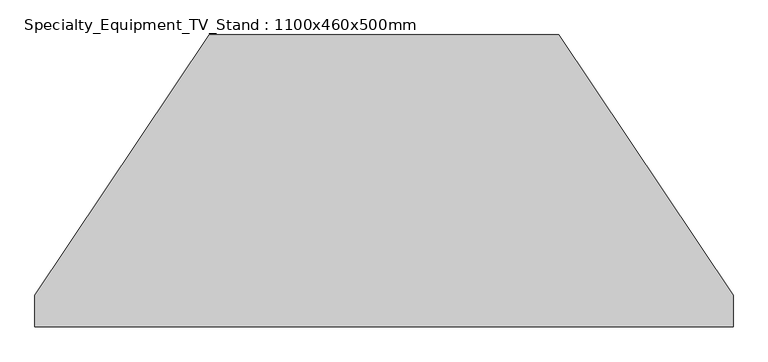
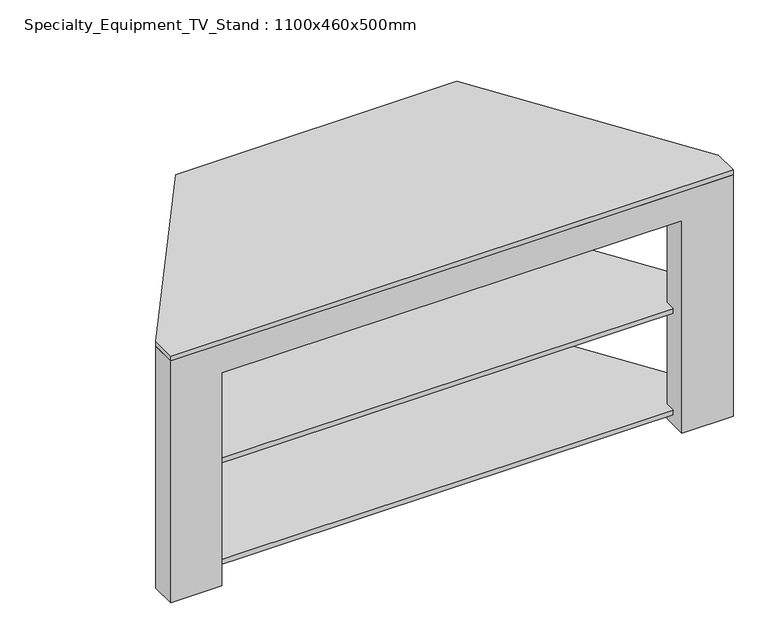
"""IFC4 building model written with IfcOpenShell, lengths in millimetres: proxy geometry, Specialty_Equipment_TV_Stand : 1100x460x500mm."""

import ifcopenshell
import ifcopenshell.guid

model = None  # the IFC model being written
_history = None  # IfcOwnerHistory: only IFC2X3 demands one
_inside = {}  # id of a spatial element -> (the spatial element, [elements in it])
_under = {}  # id of a project, library or spatial element -> (it, [spatial elements below it])
_declared = {}  # id of a project -> (the project, [libraries it declares])
_typed = {}  # id of a type object -> (the type object, [elements of that type])
_made_of = {}  # id of a material, layer set ... -> (it, [elements and type objects made of it])


def new_model(schema):
    """Start an empty IFC model of exactly this schema.

    Asked for "IFC4X3", IfcOpenShell would pick the latest addendum, in which some entities
    have other attributes; the version numbers below select the first issue.
    IFC2X3 requires an IfcOwnerHistory on every rooted entity: one is made here for all.
    """
    global model, _history
    if schema == "IFC4X3":
        model = ifcopenshell.file(schema_version=(4, 3, 0, 0))
    else:
        model = ifcopenshell.file(schema=schema)
    _inside.clear()
    _under.clear()
    _declared.clear()
    _typed.clear()
    _made_of.clear()
    _history = None
    if model.schema == "IFC2X3":
        org = make("IfcOrganization", Name="unknown")
        user = make(
            "IfcPersonAndOrganization",
            ThePerson=make("IfcPerson", FamilyName="unknown"),
            TheOrganization=org,
        )
        app = make(
            "IfcApplication",
            ApplicationDeveloper=org,
            Version="unknown",
            ApplicationFullName="unknown",
            ApplicationIdentifier="unknown",
        )
        _history = make(
            "IfcOwnerHistory",
            OwningUser=user,
            OwningApplication=app,
            ChangeAction="ADDED",
            CreationDate=0,
        )
    return model


def make(cls, **values):
    """One entity of the class cls with the attributes given. An attribute that is None is left unset."""
    return model.create_entity(
        cls, **{name: value for name, value in values.items() if value is not None}
    )


def rooted(cls, **values):
    """An entity with a GlobalId (a new one), such as an element, a storey or a relation."""
    return make(cls, GlobalId=ifcopenshell.guid.new(), OwnerHistory=_history, **values)


def si_unit(unit_type, name, prefix=None):
    """IfcSIUnit, for example si_unit("LENGTHUNIT", "METRE", prefix="MILLI")."""
    return make("IfcSIUnit", UnitType=unit_type, Prefix=prefix, Name=name)


def assignment(units):
    """IfcUnitAssignment: the units of a project."""
    return None if units is None else make("IfcUnitAssignment", Units=units)


def point(xyz):
    """IfcCartesianPoint."""
    return None if xyz is None else make("IfcCartesianPoint", Coordinates=xyz)


def direction(xyz):
    """IfcDirection."""
    return None if xyz is None else make("IfcDirection", DirectionRatios=xyz)


def frame(location, z_axis=None, x_axis=None):
    """IfcAxis2Placement3D, a coordinate frame: its origin and axes. An axis left out is left unset."""
    return make(
        "IfcAxis2Placement3D",
        Location=point(location),
        Axis=direction(z_axis),
        RefDirection=direction(x_axis),
    )


def frame_2d(location, x_axis=None):
    """IfcAxis2Placement2D, a coordinate frame in the plane: its origin and x axis."""
    return make(
        "IfcAxis2Placement2D", Location=point(location), RefDirection=direction(x_axis)
    )


def origin():
    """The frame at (0, 0, 0) with its axes left unset."""
    return frame((0.0, 0.0, 0.0))


def place(relative_to, where):
    """IfcLocalPlacement: puts the frame where relative to a parent placement (None: the world)."""
    return make(
        "IfcLocalPlacement", PlacementRelTo=relative_to, RelativePlacement=where
    )


def context(
    kind, dimensions, precision=None, world=None, true_north=None, identifier=None
):
    """IfcGeometricRepresentationContext, for example the 3D "Model" context."""
    return make(
        "IfcGeometricRepresentationContext",
        ContextIdentifier=identifier,
        ContextType=kind,
        CoordinateSpaceDimension=dimensions,
        Precision=precision,
        WorldCoordinateSystem=world,
        TrueNorth=true_north,
    )


def project(units=None, contexts=None):
    """IfcProject with its units and contexts."""
    return rooted(
        "IfcProject",
        Name="project",
        RepresentationContexts=contexts,
        UnitsInContext=assignment(units),
    )


def spatial(cls, under=None, at=None, **own):
    """A site, building, storey or space (cls), placed at a placement, below another one or the project."""
    s = rooted(cls, ObjectPlacement=at, **own)
    if under is not None:
        _under.setdefault(under.id(), (under, []))[1].append(s)
    return s


def polyline(points):
    """IfcPolyline through the points."""
    return make("IfcPolyline", Points=[point(p) for p in points])


def circle_curve(where, radius):
    """IfcCircle in the frame where."""
    return make("IfcCircle", Position=where, Radius=radius)


def trimmed(basis, trim1, trim2, sense, master):
    """IfcTrimmedCurve: the piece of a basis curve between two trims."""
    return make(
        "IfcTrimmedCurve",
        BasisCurve=basis,
        Trim1=trim1,
        Trim2=trim2,
        SenseAgreement=sense,
        MasterRepresentation=master,
    )


def segment(curve, same_sense, transition):
    """IfcCompositeCurveSegment."""
    return make(
        "IfcCompositeCurveSegment",
        Transition=transition,
        SameSense=same_sense,
        ParentCurve=curve,
    )


def composite_curve(segments, self_intersect=None):
    """IfcCompositeCurve: segments joined end to end."""
    return make("IfcCompositeCurve", Segments=segments, SelfIntersect=self_intersect)


def outline(outer, holes=None, kind="AREA"):
    """IfcArbitraryClosedProfileDef: a profile drawn as a closed curve; with holes, ...WithVoids."""
    if holes is None:
        return make("IfcArbitraryClosedProfileDef", ProfileType=kind, OuterCurve=outer)
    return make(
        "IfcArbitraryProfileDefWithVoids",
        ProfileType=kind,
        OuterCurve=outer,
        InnerCurves=holes,
    )


def extrude(swept, where, along, depth):
    """IfcExtrudedAreaSolid: the profile swept, set in the frame where, extruded along a direction by depth."""
    return make(
        "IfcExtrudedAreaSolid",
        SweptArea=swept,
        Position=where,
        ExtrudedDirection=direction(along),
        Depth=depth,
    )


def faces_of(points, faces, orient=None, outer=None):
    """IfcFace entities. A face is a list of loops; a loop is a list of indices into points, from 0.

    orient and outer hold one flag for each loop. By default every Orientation is true, the
    first loop of a face is its IfcFaceOuterBound and the others are IfcFaceBound.
    """
    made = []
    for i, loops in enumerate(faces):
        bounds = []
        for j, loop in enumerate(loops):
            is_outer = j == 0 if outer is None else outer[i][j]
            bounds.append(
                make(
                    "IfcFaceOuterBound" if is_outer else "IfcFaceBound",
                    Bound=make("IfcPolyLoop", Polygon=[points[k] for k in loop]),
                    Orientation=True if orient is None else orient[i][j],
                )
            )
        made.append(make("IfcFace", Bounds=bounds))
    return made


def faceted_brep(points, faces, orient=None, outer=None, voids=None):
    """IfcFacetedBrep: a solid bounded by flat faces; with voids (closed shells), ...WithVoids."""
    shared = [point(p) for p in points]
    hull = make("IfcClosedShell", CfsFaces=faces_of(shared, faces, orient, outer))
    if voids is None:
        return make("IfcFacetedBrep", Outer=hull)
    return make(
        "IfcFacetedBrepWithVoids",
        Outer=hull,
        Voids=[
            make(cls, CfsFaces=faces_of(shared, fs, o, b)) for cls, fs, o, b in voids
        ],
    )


def shape(context_of_items, identifier, shape_type, items):
    """IfcShapeRepresentation: the items that make up one representation, for example the "Body"."""
    return make(
        "IfcShapeRepresentation",
        ContextOfItems=context_of_items,
        RepresentationIdentifier=identifier,
        RepresentationType=shape_type,
        Items=items,
    )


def source(mapping_origin, context_of_items, identifier, shape_type, items):
    """IfcRepresentationMap: a shape defined once, which mapped items show again and again."""
    return make(
        "IfcRepresentationMap",
        MappingOrigin=mapping_origin,
        MappedRepresentation=shape(context_of_items, identifier, shape_type, items),
    )


def transform(
    local_origin,
    x_axis=None,
    y_axis=None,
    z_axis=None,
    scale=None,
    scale2=None,
    scale3=None,
    uniform=True,
):
    """IfcCartesianTransformationOperator3D, or its non-uniform kind. x_axis, y_axis, z_axis: its Axis1, 2, 3."""
    if uniform:
        return make(
            "IfcCartesianTransformationOperator3D",
            Axis1=direction(x_axis),
            Axis2=direction(y_axis),
            LocalOrigin=point(local_origin),
            Scale=scale,
            Axis3=direction(z_axis),
        )
    return make(
        "IfcCartesianTransformationOperator3DnonUniform",
        Axis1=direction(x_axis),
        Axis2=direction(y_axis),
        LocalOrigin=point(local_origin),
        Scale=scale,
        Axis3=direction(z_axis),
        Scale2=scale2,
        Scale3=scale3,
    )


def mapped(mapping_source, mapping_target):
    """IfcMappedItem: shows the shape of a source again, moved by a transform."""
    return make(
        "IfcMappedItem", MappingSource=mapping_source, MappingTarget=mapping_target
    )


def made_of(thing, what):
    """Note that an element or type object is made of a material, layer set ...; save() writes the relation."""
    if what is not None:
        _made_of.setdefault(what.id(), (what, []))[1].append(thing)
    return thing


def element(
    cls,
    number,
    at=None,
    inside=None,
    cuts=None,
    type_object=None,
    material=None,
    context=None,
    identifier="Body",
    shape_type=None,
    held_by="IfcProductDefinitionShape",
    body=None,
    shapes=None,
    **own,
):
    """One element of the class cls, such as IfcWall. Its Tag is "e" and its number.

    at: its placement. inside: the storey or other place that contains it. cuts: it is an
    opening in that element (IfcRelVoidsElement). A single representation is given by context,
    identifier, shape_type and body (its items); several are given by shapes. held_by: the class
    of the entity that holds the representations. save() writes the other relations.
    """
    e = rooted(cls, Tag="e%d" % number, ObjectPlacement=at, **own)
    if body is not None:
        shapes = [shape(context, identifier, shape_type, body)]
    if shapes is not None:
        e.Representation = make(held_by, Representations=shapes)
    if inside is not None:
        _inside.setdefault(inside.id(), (inside, []))[1].append(e)
    if cuts is not None:
        rooted(
            "IfcRelVoidsElement", RelatingBuildingElement=cuts, RelatedOpeningElement=e
        )
    if type_object is not None:
        _typed.setdefault(type_object.id(), (type_object, []))[1].append(e)
    return made_of(e, material)


def aggregate(whole, parts):
    """IfcRelAggregates: a whole, such as a stair, and the parts it consists of."""
    return rooted("IfcRelAggregates", RelatingObject=whole, RelatedObjects=parts)


def save(model, path):
    """Write the relations noted so far, then the file.

    IfcRelAggregates (storeys below a building ...), IfcRelContainedInSpatialStructure (elements
    in a storey), IfcRelDefinesByType, IfcRelAssociatesMaterial and IfcRelDeclares: one each for
    every whole, place, type object, material and project.
    """
    for whole, parts in _under.values():
        aggregate(whole, parts)
    for where, things in _inside.values():
        rooted(
            "IfcRelContainedInSpatialStructure",
            RelatedElements=things,
            RelatingStructure=where,
        )
    for kind, things in _typed.values():
        rooted("IfcRelDefinesByType", RelatedObjects=things, RelatingType=kind)
    for what, things in _made_of.values():
        rooted("IfcRelAssociatesMaterial", RelatedObjects=things, RelatingMaterial=what)
    for by, libraries in _declared.values():
        rooted("IfcRelDeclares", RelatingContext=by, RelatedDefinitions=libraries)
    model.write(path)


def specialty_equipment_tv_stand_1100x460x500mm_40ec15d9(model_context):
    return source(origin(), model_context, "Body", "SolidModel", [
        extrude(outline(polyline([(420.3099533, -30.0), (625.1880021, -335.4545455), (625.1880021, -430.0), (-374.8119979, -430.0), (-374.8119979, -335.4545455), (-169.9339492, -30.0), (420.3099533, -30.0)])), frame((0.0, 0.0, 20.0), z_axis=(0.0, 0.0, 1.0), x_axis=(1.0, 0.0, 0.0)), (0.0, 0.0, 1.0), 10.0),
        extrude(outline(polyline([(420.3099533, -30.0), (625.1880021, -335.4545455), (625.1880021, -430.0), (-374.8119979, -430.0), (-374.8119979, -335.4545455), (-169.9339492, -30.0), (420.3099533, -30.0)])), frame((0.0, 0.0, 230.0), z_axis=(0.0, 0.0, 1.0), x_axis=(1.0, 0.0, 0.0)), (0.0, 0.0, 1.0), 10.0),
        extrude(outline(polyline([(400.1880021, 0.0), (675.1880021, -410.0), (675.1880021, -460.0), (-424.8119979, -460.0), (-424.8119979, -410.0), (-149.8119979, 0.0), (400.1880021, 0.0)])), frame((0.0, 0.0, 500.0), z_axis=(0.0, 0.0, 1.0), x_axis=(1.0, 0.0, 0.0)), (0.0, 0.0, 1.0), 10.0),
        extrude(outline(polyline([(-50.0, 500.0), (0.0, 500.0), (0.0, 0.0), (-50.0, 0.0), (-50.0, 20.0), (-30.0, 20.0), (-30.0, 30.0), (-50.0, 30.0), (-50.0, 230.0), (-30.0, 230.0), (-30.0, 240.0), (-50.0, 240.0), (-50.0, 500.0)])), frame((-149.8119979, 0.0, 0.0), z_axis=(1.0, 0.0, 0.0), x_axis=(0.0, 1.0, 0.0)), (0.0, 0.0, 1.0), 100.0),
        extrude(outline(polyline([(-50.0, 500.0), (0.0, 500.0), (0.0, 0.0), (-50.0, 0.0), (-50.0, 20.0), (-30.0, 20.0), (-30.0, 30.0), (-50.0, 30.0), (-50.0, 230.0), (-30.0, 230.0), (-30.0, 240.0), (-50.0, 240.0), (-50.0, 500.0)])), frame((300.1880021, 0.0, 0.0), z_axis=(1.0, 0.0, 0.0), x_axis=(0.0, 1.0, 0.0)), (0.0, 0.0, 1.0), 100.0),
        faceted_brep([(-424.8119979, -460.0, 0.0), (-324.8119979, -460.0, 0.0), (-324.8119979, -460.0, 440.0), (575.1880021, -460.0, 440.0), (575.1880021, -460.0, 0.0), (675.1880021, -460.0, 0.0), (675.1880021, -460.0, 500.0), (-424.8119979, -460.0, 500.0), (-424.8119979, -410.0, 0.0), (-424.8119979, -410.0, 500.0), (675.1880021, -410.0, 500.0), (675.1880021, -410.0, 0.0), (575.1880021, -410.0, 0.0), (575.1880021, -410.0, 20.0), (625.1880021, -410.0, 20.0), (625.1880021, -410.0, 30.0), (575.1880021, -410.0, 30.0), (575.1880021, -410.0, 230.0), (625.1880021, -410.0, 230.0), (625.1880021, -410.0, 240.0), (575.1880021, -410.0, 240.0), (575.1880021, -410.0, 440.0), (-324.8119979, -410.0, 440.0), (-324.8119979, -410.0, 240.0), (-374.8119979, -410.0, 240.0), (-374.8119979, -410.0, 230.0), (-324.8119979, -410.0, 230.0), (-324.8119979, -410.0, 30.0), (-374.8119979, -410.0, 30.0), (-374.8119979, -410.0, 20.0), (-324.8119979, -410.0, 20.0), (-324.8119979, -410.0, 0.0), (-324.8119979, -430.0, 20.0), (-324.8119979, -430.0, 30.0), (-324.8119979, -430.0, 230.0), (-324.8119979, -430.0, 240.0), (575.1880021, -430.0, 240.0), (575.1880021, -430.0, 230.0), (575.1880021, -430.0, 30.0), (575.1880021, -430.0, 20.0), (625.1880021, -430.0, 240.0), (-374.8119979, -430.0, 240.0), (-374.8119979, -430.0, 230.0), (625.1880021, -430.0, 230.0), (625.1880021, -430.0, 30.0), (-374.8119979, -430.0, 30.0), (-374.8119979, -430.0, 20.0), (625.1880021, -430.0, 20.0)], [[[0, 1, 2, 3, 4, 5, 6, 7]], [[8, 9, 10, 11, 12, 13, 14, 15, 16, 17, 18, 19, 20, 21, 22, 23, 24, 25, 26, 27, 28, 29, 30, 31]], [[1, 0, 8, 31]], [[2, 1, 31, 30, 32, 33, 27, 26, 34, 35, 23, 22]], [[3, 2, 22, 21]], [[4, 3, 21, 20, 36, 37, 17, 16, 38, 39, 13, 12]], [[5, 4, 12, 11]], [[6, 5, 11, 10]], [[7, 6, 10, 9]], [[0, 7, 9, 8]], [[19, 40, 36, 20]], [[35, 41, 24, 23]], [[25, 42, 34, 26]], [[37, 43, 18, 17]], [[41, 42, 25, 24]], [[42, 41, 35, 34]], [[40, 43, 37, 36]], [[43, 40, 19, 18]], [[15, 44, 38, 16]], [[33, 45, 28, 27]], [[29, 46, 32, 30]], [[39, 47, 14, 13]], [[45, 46, 29, 28]], [[46, 45, 33, 32]], [[44, 47, 39, 38]], [[47, 44, 15, 14]]]),
        extrude(outline(polyline([(0.0, 300.1880021), (500.0, 300.1880021), (500.0, -49.8119979), (0.0, -49.8119979), (0.0, 300.1880021)]), holes=[composite_curve([segment(polyline([(245.0, 145.1700818), (245.0, 105.2059224)]), True, "CONTINUOUS"), segment(trimmed(circle_curve(frame_2d((257.5, 105.2059224)), 12.5), [point((245.0, 105.2059224))], [point((270.0, 105.2059224))], True, "CARTESIAN"), True, "CONTINUOUS"), segment(polyline([(270.0, 105.2059224), (270.0, 145.1700818)]), True, "CONTINUOUS"), segment(trimmed(circle_curve(frame_2d((257.5, 145.1700818)), 12.5), [point((270.0, 145.1700818))], [point((245.0, 145.1700818))], True, "CARTESIAN"), True, "CONTINUOUS")], self_intersect=False), composite_curve([segment(polyline([(35.0, 145.1880021), (35.0, 105.2059224)]), True, "CONTINUOUS"), segment(trimmed(circle_curve(frame_2d((47.5, 105.2059224)), 12.5), [point((35.0, 105.2059224))], [point((60.0, 105.2059224))], True, "CARTESIAN"), True, "CONTINUOUS"), segment(polyline([(60.0, 105.2059224), (60.0, 145.1880021)]), True, "CONTINUOUS"), segment(trimmed(circle_curve(frame_2d((47.5, 145.1880021)), 12.5), [point((60.0, 145.1880021))], [point((35.0, 145.1880021))], True, "CARTESIAN"), True, "CONTINUOUS")], self_intersect=False)]), frame((0.0, -30.0, 0.0), z_axis=(0.0, 1.0, 0.0), x_axis=(0.0, 0.0, 1.0)), (0.0, 0.0, 1.0), 10.0),
    ])


if __name__ == "__main__":
    model = new_model("IFC4")
    model_context = context("Model", 3, world=origin())
    ifc_project = project(units=[si_unit("LENGTHUNIT", "METRE", prefix="MILLI")], contexts=[model_context])
    site = spatial("IfcSite", under=ifc_project)
    building = spatial("IfcBuilding", under=site)
    placement = place(None, origin())
    specialty_equipment_tv_stand_1100x460x500mm_shape = specialty_equipment_tv_stand_1100x460x500mm_40ec15d9(model_context)
    element("IfcBuildingElementProxy", 1, Name="Specialty_Equipment_TV_Stand : 1100x460x500mm", ObjectType="Specialty_Equipment_TV_Stand : 1100x460x500mm", at=placement, inside=building, context=model_context, shape_type="MappedRepresentation", body=[
        mapped(specialty_equipment_tv_stand_1100x460x500mm_shape, transform((0.0, 0.0, 0.0), x_axis=(1.0, 0.0, 0.0), y_axis=(0.0, 1.0, 0.0), z_axis=(0.0, 0.0, 1.0))),
    ])
    save(model, "model.ifc")

# Revit data of these elements
# Type "Specialty_Equipment_TV_Stand : 1100x460x500mm"
#   Depth = 460 mm
#   Width = 1100 mm
#   Height = 500 mm
#   Finish = Melamine - Gray
# Element 1 (IfcBuildingElementProxy, "Specialty_Equipment_TV_Stand : 1100x460x500mm")
#   Materials on its faces: "Melamine - Gray", "Glass - Shelves"
# Materials
#   "Melamine - Gray": class "Wood", colour RGB 49 49 49, transparency 0
#   "Glass - Shelves": class "Glass", colour RGB 167 167 167, transparency 0.9
